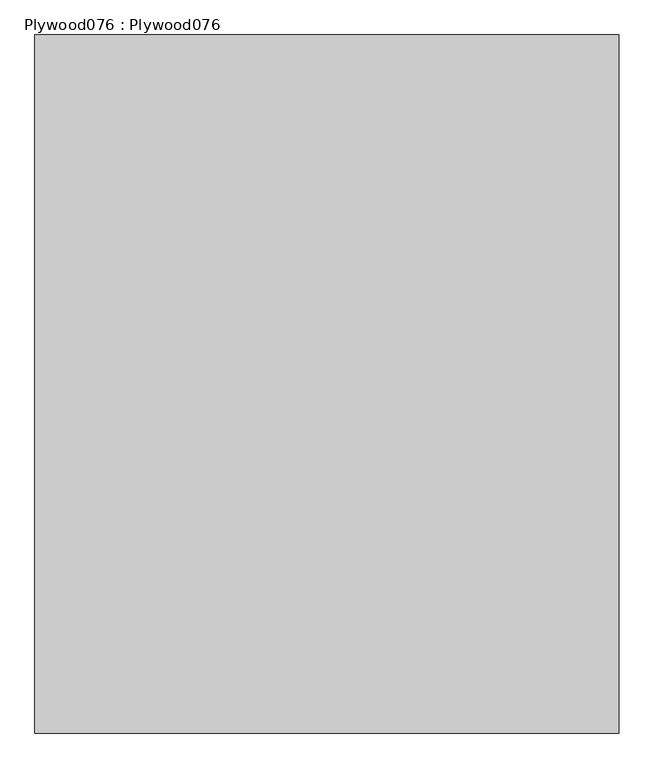
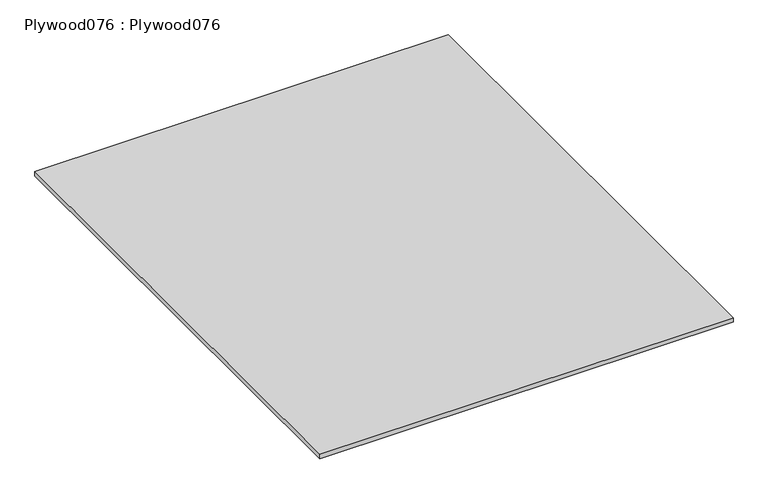
"""IFC4 building model written with IfcOpenShell, lengths in millimetres: proxy geometry, Plywood076 : Plywood076."""

from ifc_helpers import new_model, si_unit, frame, origin, place, context, project, spatial, polyline, outline, extrude, source, transform, mapped, element, save


def plywood076_plywood076_dc0197f9(model_context):
    return source(origin(), model_context, "Body", "SweptSolid", [
        extrude(outline(polyline([(-1090.0815411, -1052.8906574), (-2764.2237014, -1052.8906574), (-2764.2237014, 947.1093426), (-1090.0815411, 947.1093426), (-1090.0815411, -1052.8906574)])), frame((0.0, 0.0, 40112.696), z_axis=(0.0, 0.0, 1.0), x_axis=(1.0, 0.0, 0.0)), (0.0, 0.0, 1.0), 19.05),
    ])


if __name__ == "__main__":
    model = new_model("IFC4")
    model_context = context("Model", 3, world=origin())
    ifc_project = project(units=[si_unit("LENGTHUNIT", "METRE", prefix="MILLI")], contexts=[model_context])
    site = spatial("IfcSite", under=ifc_project)
    building = spatial("IfcBuilding", under=site)
    placement = place(None, origin())
    plywood076_plywood076_shape = plywood076_plywood076_dc0197f9(model_context)
    element("IfcBuildingElementProxy", 1, Name="Plywood076 : Plywood076", ObjectType="Plywood076 : Plywood076", at=placement, inside=building, context=model_context, shape_type="MappedRepresentation", body=[
        mapped(plywood076_plywood076_shape, transform((0.0, 0.0, 0.0), x_axis=(1.0, 0.0, 0.0), y_axis=(0.0, 1.0, 0.0), z_axis=(0.0, 0.0, 1.0))),
    ])
    save(model, "model.ifc")

# Revit data of these elements
# Type "Plywood076 : Plywood076"
#   NameOverride = "Plywood076"
# Element 1 (IfcBuildingElementProxy, "Plywood076 : Plywood076")
#   Materials on its faces: "CDX PLYWOOD -  SEE STRUCTURAL DWGS"
# Materials
#   "CDX PLYWOOD -  SEE STRUCTURAL DWGS": class "Unassigned", colour RGB 177 130 114, transparency 0, Cost = 0
